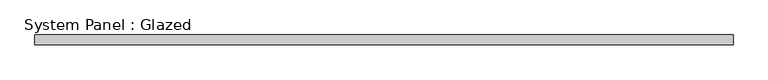
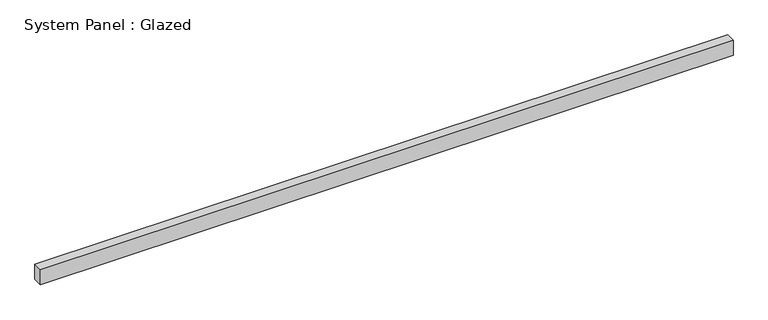
"""IFC4 building model written with IfcOpenShell, lengths in millimetres: plate geometry, System Panel : Glazed."""

from ifc_helpers import new_model, si_unit, origin, origin_with_axes, place, context, project, spatial, polyline, outline, extrude, source, transform, mapped, element, save


def system_panel_glazed_7f82afe2(model_context):
    return source(origin(), model_context, "Body", "SweptSolid", [
        extrude(outline(polyline([(914.4, -44.45), (-914.4, -44.45), (-914.4, -19.05), (914.4, -19.05), (914.4, -44.45)])), origin_with_axes(), (0.0, 0.0, 1.0), 41.9143134),
    ])


if __name__ == "__main__":
    model = new_model("IFC4")
    model_context = context("Model", 3, world=origin())
    ifc_project = project(units=[si_unit("LENGTHUNIT", "METRE", prefix="MILLI")], contexts=[model_context])
    site = spatial("IfcSite", under=ifc_project)
    building = spatial("IfcBuilding", under=site)
    placement = place(None, origin())
    system_panel_glazed_shape = system_panel_glazed_7f82afe2(model_context)
    element("IfcPlate", 1, ObjectType="System Panel : Glazed", at=placement, inside=building, context=model_context, shape_type="MappedRepresentation", body=[
        mapped(system_panel_glazed_shape, transform((0.0, 0.0, 0.0), x_axis=(1.0, 0.0, 0.0), y_axis=(0.0, 1.0, 0.0), z_axis=(0.0, 0.0, 1.0))),
    ])
    save(model, "model.ifc")

# Revit data of these elements
# Type "System Panel : Glazed"
#   Construction Type Id = "GSP4R"
#   Analytic Construction = "1/8 in Pilkington single glazing"
#   Visual Light Transmittance = 0.9
#   Solar Heat Gain Coefficient = 0.86
#   Heat Transfer Coefficient (U) = 1.18115 BTU/(h·ft²·°F)
#   Define Thermal Properties by = 1
# Element 1 (IfcPlate, "System Panel : Glazed")
#   Materials on its faces: "Glass"
# Materials
#   "Glass": class "Glass", colour RGB 0 128 192, transparency 0.75, Description = "Soda Lime Glass", Cost = 0
